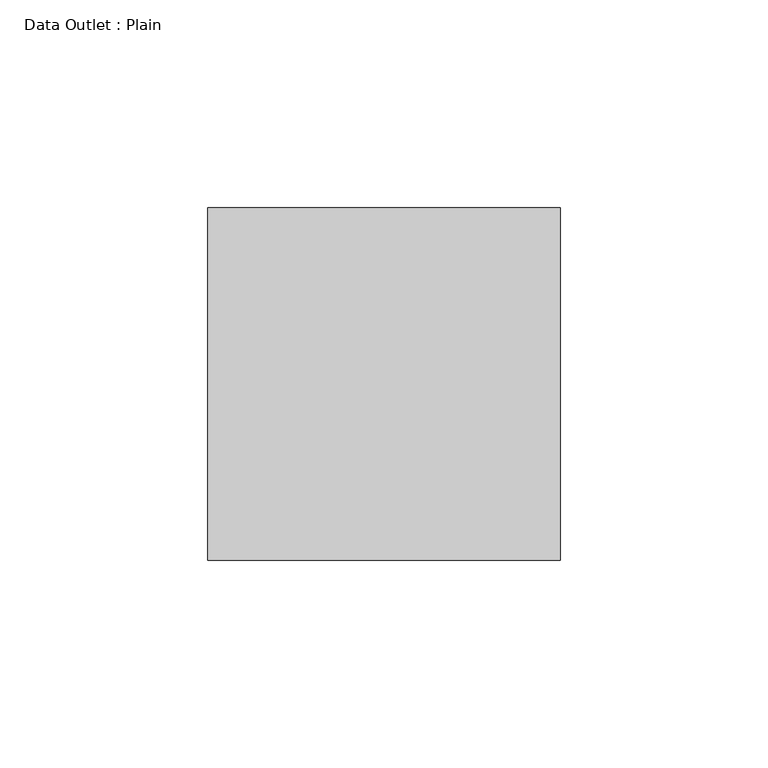
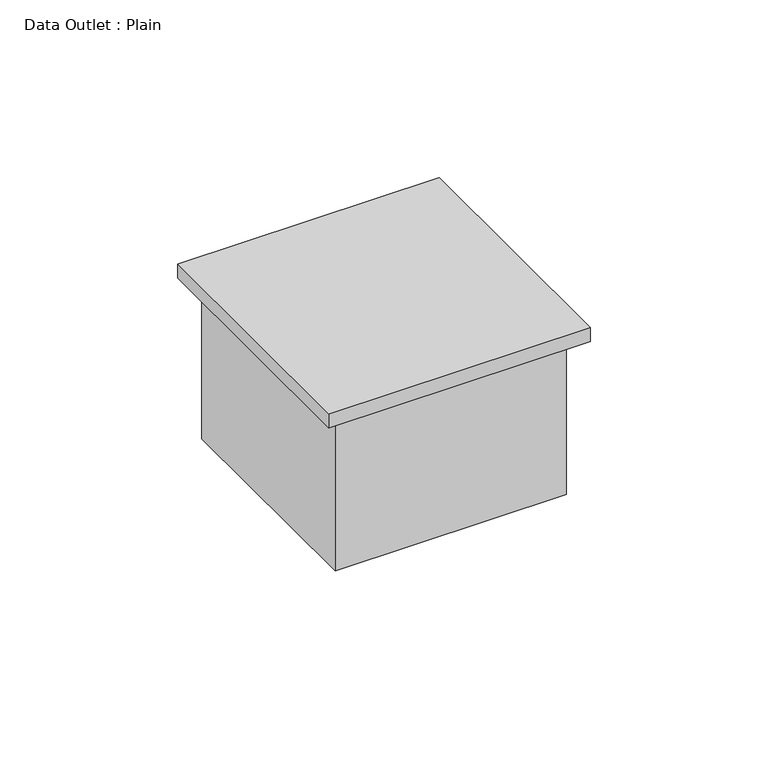
"""IFC4 building model written with IfcOpenShell, lengths in millimetres: electric appliance geometry, Data Outlet : Plain."""

from ifc_helpers import new_model, si_unit, frame, origin, origin_with_axes, place, context, project, spatial, polyline, outline, extrude, source, transform, mapped, element, save


def data_outlet_plain_4a0886d3(model_context):
    return source(origin(), model_context, "Body", "SweptSolid", [
        extrude(outline(polyline([(42.5, 42.5), (42.5, -42.5), (-42.5, -42.5), (-42.5, 42.5), (42.5, 42.5)])), origin_with_axes(), (0.0, 0.0, 1.0), 4.7625),
        extrude(outline(polyline([(37.5, 37.5), (37.5, -37.5), (-37.5, -37.5), (-37.5, 37.5), (37.5, 37.5)])), frame((0.0, 0.0, -53.975), z_axis=(0.0, 0.0, 1.0), x_axis=(1.0, 0.0, 0.0)), (0.0, 0.0, 1.0), 53.975),
    ])


if __name__ == "__main__":
    model = new_model("IFC4")
    model_context = context("Model", 3, world=origin())
    ifc_project = project(units=[si_unit("LENGTHUNIT", "METRE", prefix="MILLI")], contexts=[model_context])
    site = spatial("IfcSite", under=ifc_project)
    building = spatial("IfcBuilding", under=site)
    placement = place(None, origin())
    data_outlet_plain_shape = data_outlet_plain_4a0886d3(model_context)
    element("IfcElectricAppliance", 1, ObjectType="Data Outlet : Plain", at=placement, inside=building, context=model_context, shape_type="MappedRepresentation", body=[
        mapped(data_outlet_plain_shape, transform((0.0, 0.0, 0.0), x_axis=(1.0, 0.0, 0.0), y_axis=(0.0, 1.0, 0.0), z_axis=(0.0, 0.0, 1.0))),
    ])
    save(model, "model.ifc")

# Revit data of these elements
# Type "Data Outlet : Plain"
#   Label = "D"
#   Default Elevation = 460 mm
#   Assembly Code = ""
